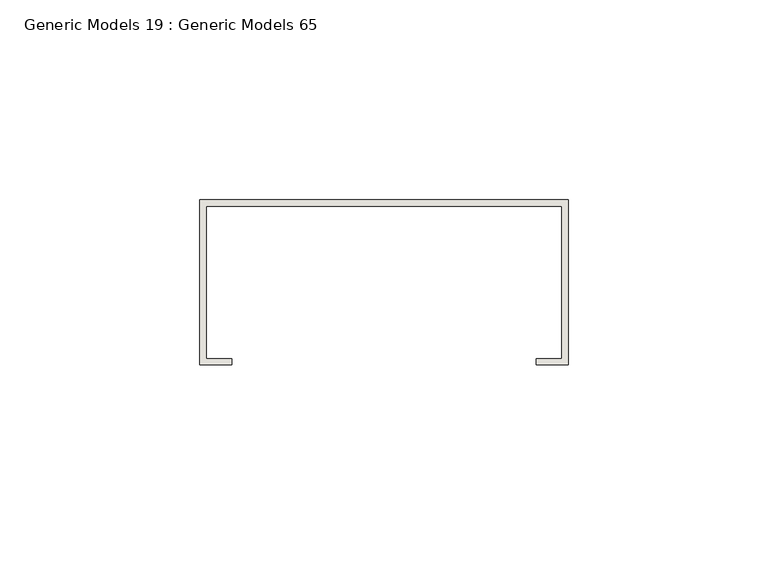
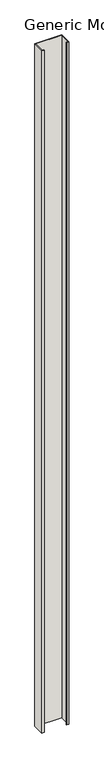
"""IFC4 building model written with IfcOpenShell, lengths in millimetres: wall geometry, Generic Models 19 : Generic Models 65."""

from ifc_helpers import new_model, si_unit, frame, origin, place, context, project, spatial, polyline, outline, extrude, source, transform, mapped, element, save


def generic_models_19_generic_models_65_4a0df7f0(model_context):
    return source(origin(), model_context, "Body", "SweptSolid", [
        extrude(outline(polyline([(49691.925, 630.2375), (49784.0, 630.2375), (49784.0, 588.9625), (49776.0625, 588.9625), (49776.0625, 590.55), (49782.4125, 590.55), (49782.4125, 628.65), (49693.5125, 628.65), (49693.5125, 590.55), (49699.8625, 590.55), (49699.8625, 588.9625), (49691.925, 588.9625), (49691.925, 630.2375)])), frame((0.0, 0.0, 1.5875), z_axis=(0.0, 0.0, 1.0), x_axis=(1.0, 0.0, 0.0)), (0.0, 0.0, 1.0), 2454.275),
    ])


if __name__ == "__main__":
    model = new_model("IFC4")
    model_context = context("Model", 3, world=origin())
    ifc_project = project(units=[si_unit("LENGTHUNIT", "METRE", prefix="MILLI")], contexts=[model_context])
    site = spatial("IfcSite", under=ifc_project)
    building = spatial("IfcBuilding", under=site)
    placement = place(None, origin())
    generic_models_19_generic_models_65_shape = generic_models_19_generic_models_65_4a0df7f0(model_context)
    element("IfcWall", 1, ObjectType="Generic Models 19 : Generic Models 65", at=placement, inside=building, context=model_context, shape_type="MappedRepresentation", body=[
        mapped(generic_models_19_generic_models_65_shape, transform((0.0, 0.0, 0.0), x_axis=(1.0, 0.0, 0.0), y_axis=(0.0, 1.0, 0.0), z_axis=(0.0, 0.0, 1.0))),
    ])
    save(model, "model.ifc")

# Revit data of these elements
# Element 1 (IfcWall, "Generic Models 19 : Generic Models 65")
#   Materials on its faces: "METAL STUDS - SEE 'WALL TAG' & 'LAYER MATERIAL SCHEDULE' FOR GAUGE/SPACING & INSULATION TREATMENT, IF APPLICABLE"
# Materials
#   "METAL STUDS - SEE 'WALL TAG' & 'LAYER MATERIAL SCHEDULE' FOR GAUGE/SPACING & INSULATION TREATMENT, IF APPLICABLE": class "Unassigned", colour RGB 210 209 208, transparency 0, Keynote = "M05121300.02", Cost = 0
